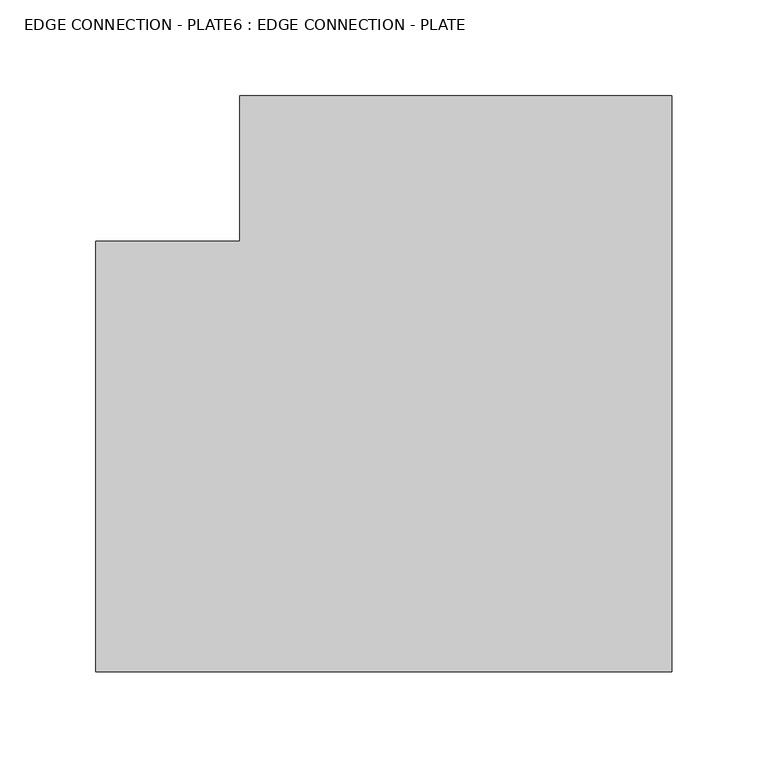
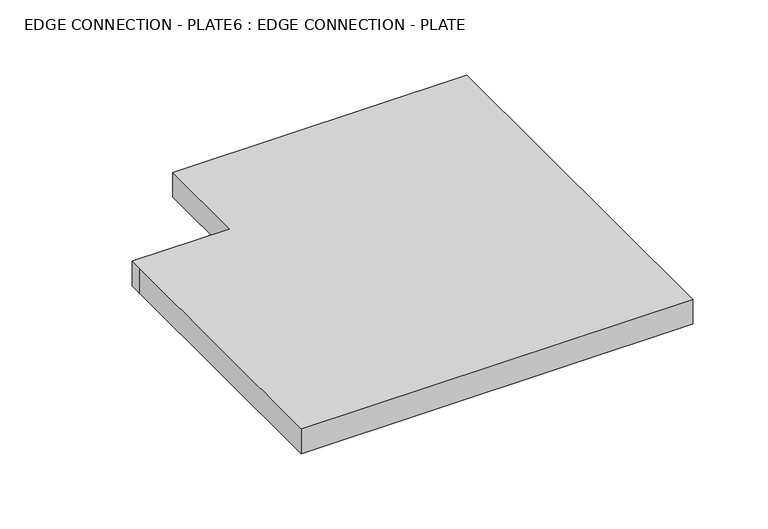
"""IFC4 building model written with IfcOpenShell, lengths in millimetres: fastener geometry, EDGE CONNECTION - PLATE6 : EDGE CONNECTION - PLATE."""

import ifcopenshell
import ifcopenshell.guid

model = None  # the IFC model being written
_history = None  # IfcOwnerHistory: only IFC2X3 demands one
_inside = {}  # id of a spatial element -> (the spatial element, [elements in it])
_under = {}  # id of a project, library or spatial element -> (it, [spatial elements below it])
_declared = {}  # id of a project -> (the project, [libraries it declares])
_typed = {}  # id of a type object -> (the type object, [elements of that type])
_made_of = {}  # id of a material, layer set ... -> (it, [elements and type objects made of it])


def new_model(schema):
    """Start an empty IFC model of exactly this schema.

    Asked for "IFC4X3", IfcOpenShell would pick the latest addendum, in which some entities
    have other attributes; the version numbers below select the first issue.
    IFC2X3 requires an IfcOwnerHistory on every rooted entity: one is made here for all.
    """
    global model, _history
    if schema == "IFC4X3":
        model = ifcopenshell.file(schema_version=(4, 3, 0, 0))
    else:
        model = ifcopenshell.file(schema=schema)
    _inside.clear()
    _under.clear()
    _declared.clear()
    _typed.clear()
    _made_of.clear()
    _history = None
    if model.schema == "IFC2X3":
        org = make("IfcOrganization", Name="unknown")
        user = make(
            "IfcPersonAndOrganization",
            ThePerson=make("IfcPerson", FamilyName="unknown"),
            TheOrganization=org,
        )
        app = make(
            "IfcApplication",
            ApplicationDeveloper=org,
            Version="unknown",
            ApplicationFullName="unknown",
            ApplicationIdentifier="unknown",
        )
        _history = make(
            "IfcOwnerHistory",
            OwningUser=user,
            OwningApplication=app,
            ChangeAction="ADDED",
            CreationDate=0,
        )
    return model


def make(cls, **values):
    """One entity of the class cls with the attributes given. An attribute that is None is left unset."""
    return model.create_entity(
        cls, **{name: value for name, value in values.items() if value is not None}
    )


def rooted(cls, **values):
    """An entity with a GlobalId (a new one), such as an element, a storey or a relation."""
    return make(cls, GlobalId=ifcopenshell.guid.new(), OwnerHistory=_history, **values)


def si_unit(unit_type, name, prefix=None):
    """IfcSIUnit, for example si_unit("LENGTHUNIT", "METRE", prefix="MILLI")."""
    return make("IfcSIUnit", UnitType=unit_type, Prefix=prefix, Name=name)


def assignment(units):
    """IfcUnitAssignment: the units of a project."""
    return None if units is None else make("IfcUnitAssignment", Units=units)


def point(xyz):
    """IfcCartesianPoint."""
    return None if xyz is None else make("IfcCartesianPoint", Coordinates=xyz)


def direction(xyz):
    """IfcDirection."""
    return None if xyz is None else make("IfcDirection", DirectionRatios=xyz)


def frame(location, z_axis=None, x_axis=None):
    """IfcAxis2Placement3D, a coordinate frame: its origin and axes. An axis left out is left unset."""
    return make(
        "IfcAxis2Placement3D",
        Location=point(location),
        Axis=direction(z_axis),
        RefDirection=direction(x_axis),
    )


def origin():
    """The frame at (0, 0, 0) with its axes left unset."""
    return frame((0.0, 0.0, 0.0))


def place(relative_to, where):
    """IfcLocalPlacement: puts the frame where relative to a parent placement (None: the world)."""
    return make(
        "IfcLocalPlacement", PlacementRelTo=relative_to, RelativePlacement=where
    )


def context(
    kind, dimensions, precision=None, world=None, true_north=None, identifier=None
):
    """IfcGeometricRepresentationContext, for example the 3D "Model" context."""
    return make(
        "IfcGeometricRepresentationContext",
        ContextIdentifier=identifier,
        ContextType=kind,
        CoordinateSpaceDimension=dimensions,
        Precision=precision,
        WorldCoordinateSystem=world,
        TrueNorth=true_north,
    )


def project(units=None, contexts=None):
    """IfcProject with its units and contexts."""
    return rooted(
        "IfcProject",
        Name="project",
        RepresentationContexts=contexts,
        UnitsInContext=assignment(units),
    )


def spatial(cls, under=None, at=None, **own):
    """A site, building, storey or space (cls), placed at a placement, below another one or the project."""
    s = rooted(cls, ObjectPlacement=at, **own)
    if under is not None:
        _under.setdefault(under.id(), (under, []))[1].append(s)
    return s


def polyline(points):
    """IfcPolyline through the points."""
    return make("IfcPolyline", Points=[point(p) for p in points])


def outline(outer, holes=None, kind="AREA"):
    """IfcArbitraryClosedProfileDef: a profile drawn as a closed curve; with holes, ...WithVoids."""
    if holes is None:
        return make("IfcArbitraryClosedProfileDef", ProfileType=kind, OuterCurve=outer)
    return make(
        "IfcArbitraryProfileDefWithVoids",
        ProfileType=kind,
        OuterCurve=outer,
        InnerCurves=holes,
    )


def extrude(swept, where, along, depth):
    """IfcExtrudedAreaSolid: the profile swept, set in the frame where, extruded along a direction by depth."""
    return make(
        "IfcExtrudedAreaSolid",
        SweptArea=swept,
        Position=where,
        ExtrudedDirection=direction(along),
        Depth=depth,
    )


def shape(context_of_items, identifier, shape_type, items):
    """IfcShapeRepresentation: the items that make up one representation, for example the "Body"."""
    return make(
        "IfcShapeRepresentation",
        ContextOfItems=context_of_items,
        RepresentationIdentifier=identifier,
        RepresentationType=shape_type,
        Items=items,
    )


def source(mapping_origin, context_of_items, identifier, shape_type, items):
    """IfcRepresentationMap: a shape defined once, which mapped items show again and again."""
    return make(
        "IfcRepresentationMap",
        MappingOrigin=mapping_origin,
        MappedRepresentation=shape(context_of_items, identifier, shape_type, items),
    )


def transform(
    local_origin,
    x_axis=None,
    y_axis=None,
    z_axis=None,
    scale=None,
    scale2=None,
    scale3=None,
    uniform=True,
):
    """IfcCartesianTransformationOperator3D, or its non-uniform kind. x_axis, y_axis, z_axis: its Axis1, 2, 3."""
    if uniform:
        return make(
            "IfcCartesianTransformationOperator3D",
            Axis1=direction(x_axis),
            Axis2=direction(y_axis),
            LocalOrigin=point(local_origin),
            Scale=scale,
            Axis3=direction(z_axis),
        )
    return make(
        "IfcCartesianTransformationOperator3DnonUniform",
        Axis1=direction(x_axis),
        Axis2=direction(y_axis),
        LocalOrigin=point(local_origin),
        Scale=scale,
        Axis3=direction(z_axis),
        Scale2=scale2,
        Scale3=scale3,
    )


def mapped(mapping_source, mapping_target):
    """IfcMappedItem: shows the shape of a source again, moved by a transform."""
    return make(
        "IfcMappedItem", MappingSource=mapping_source, MappingTarget=mapping_target
    )


def made_of(thing, what):
    """Note that an element or type object is made of a material, layer set ...; save() writes the relation."""
    if what is not None:
        _made_of.setdefault(what.id(), (what, []))[1].append(thing)
    return thing


def element(
    cls,
    number,
    at=None,
    inside=None,
    cuts=None,
    type_object=None,
    material=None,
    context=None,
    identifier="Body",
    shape_type=None,
    held_by="IfcProductDefinitionShape",
    body=None,
    shapes=None,
    **own,
):
    """One element of the class cls, such as IfcWall. Its Tag is "e" and its number.

    at: its placement. inside: the storey or other place that contains it. cuts: it is an
    opening in that element (IfcRelVoidsElement). A single representation is given by context,
    identifier, shape_type and body (its items); several are given by shapes. held_by: the class
    of the entity that holds the representations. save() writes the other relations.
    """
    e = rooted(cls, Tag="e%d" % number, ObjectPlacement=at, **own)
    if body is not None:
        shapes = [shape(context, identifier, shape_type, body)]
    if shapes is not None:
        e.Representation = make(held_by, Representations=shapes)
    if inside is not None:
        _inside.setdefault(inside.id(), (inside, []))[1].append(e)
    if cuts is not None:
        rooted(
            "IfcRelVoidsElement", RelatingBuildingElement=cuts, RelatedOpeningElement=e
        )
    if type_object is not None:
        _typed.setdefault(type_object.id(), (type_object, []))[1].append(e)
    return made_of(e, material)


def aggregate(whole, parts):
    """IfcRelAggregates: a whole, such as a stair, and the parts it consists of."""
    return rooted("IfcRelAggregates", RelatingObject=whole, RelatedObjects=parts)


def save(model, path):
    """Write the relations noted so far, then the file.

    IfcRelAggregates (storeys below a building ...), IfcRelContainedInSpatialStructure (elements
    in a storey), IfcRelDefinesByType, IfcRelAssociatesMaterial and IfcRelDeclares: one each for
    every whole, place, type object, material and project.
    """
    for whole, parts in _under.values():
        aggregate(whole, parts)
    for where, things in _inside.values():
        rooted(
            "IfcRelContainedInSpatialStructure",
            RelatedElements=things,
            RelatingStructure=where,
        )
    for kind, things in _typed.values():
        rooted("IfcRelDefinesByType", RelatedObjects=things, RelatingType=kind)
    for what, things in _made_of.values():
        rooted("IfcRelAssociatesMaterial", RelatedObjects=things, RelatingMaterial=what)
    for by, libraries in _declared.values():
        rooted("IfcRelDeclares", RelatingContext=by, RelatedDefinitions=libraries)
    model.write(path)


def edge_connection_plate6_edge_connection_plate_b6bb8a51(model_context):
    return source(origin(), model_context, "Body", "SweptSolid", [
        extrude(outline(polyline([(29700.0, 19499.5208589), (29700.0, 19713.9908589), (29700.0, 19723.9908589), (29774.862, 19723.9908589), (29774.862, 19799.5208589), (29784.862, 19799.5208589), (30000.0, 19799.5208589), (30000.0, 19499.5208589), (29700.0, 19499.5208589)])), frame((0.0, 0.0, 330.0), z_axis=(0.0, 0.0, 1.0), x_axis=(1.0, 0.0, 0.0)), (0.0, 0.0, 1.0), 20.0),
    ])


if __name__ == "__main__":
    model = new_model("IFC4")
    model_context = context("Model", 3, world=origin())
    ifc_project = project(units=[si_unit("LENGTHUNIT", "METRE", prefix="MILLI")], contexts=[model_context])
    site = spatial("IfcSite", under=ifc_project)
    building = spatial("IfcBuilding", under=site)
    placement = place(None, origin())
    edge_connection_plate6_edge_connection_plate_shape = edge_connection_plate6_edge_connection_plate_b6bb8a51(model_context)
    element("IfcFastener", 1, ObjectType="EDGE CONNECTION - PLATE6 : EDGE CONNECTION - PLATE", at=placement, inside=building, context=model_context, shape_type="MappedRepresentation", body=[
        mapped(edge_connection_plate6_edge_connection_plate_shape, transform((0.0, 0.0, 0.0), x_axis=(1.0, 0.0, 0.0), y_axis=(0.0, 1.0, 0.0), z_axis=(0.0, 0.0, 1.0))),
    ])
    save(model, "model.ifc")
